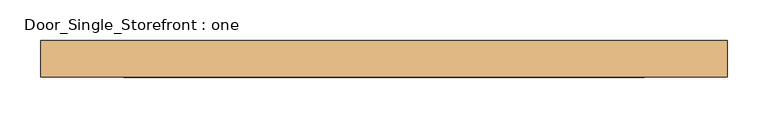
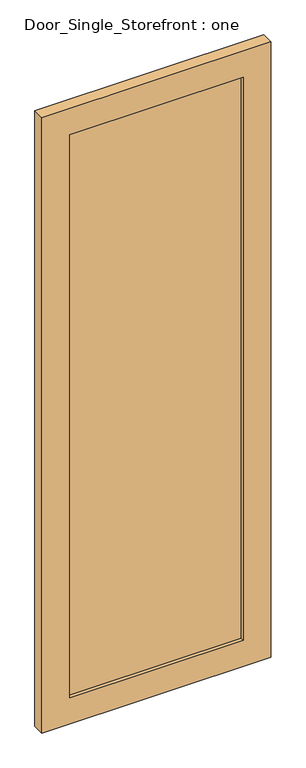
"""IFC4 building model written with IfcOpenShell, lengths in millimetres: door geometry, Door_Single_Storefront : one."""

import ifcopenshell
import ifcopenshell.guid

model = None  # the IFC model being written
_history = None  # IfcOwnerHistory: only IFC2X3 demands one
_inside = {}  # id of a spatial element -> (the spatial element, [elements in it])
_under = {}  # id of a project, library or spatial element -> (it, [spatial elements below it])
_declared = {}  # id of a project -> (the project, [libraries it declares])
_typed = {}  # id of a type object -> (the type object, [elements of that type])
_made_of = {}  # id of a material, layer set ... -> (it, [elements and type objects made of it])


def new_model(schema):
    """Start an empty IFC model of exactly this schema.

    Asked for "IFC4X3", IfcOpenShell would pick the latest addendum, in which some entities
    have other attributes; the version numbers below select the first issue.
    IFC2X3 requires an IfcOwnerHistory on every rooted entity: one is made here for all.
    """
    global model, _history
    if schema == "IFC4X3":
        model = ifcopenshell.file(schema_version=(4, 3, 0, 0))
    else:
        model = ifcopenshell.file(schema=schema)
    _inside.clear()
    _under.clear()
    _declared.clear()
    _typed.clear()
    _made_of.clear()
    _history = None
    if model.schema == "IFC2X3":
        org = make("IfcOrganization", Name="unknown")
        user = make(
            "IfcPersonAndOrganization",
            ThePerson=make("IfcPerson", FamilyName="unknown"),
            TheOrganization=org,
        )
        app = make(
            "IfcApplication",
            ApplicationDeveloper=org,
            Version="unknown",
            ApplicationFullName="unknown",
            ApplicationIdentifier="unknown",
        )
        _history = make(
            "IfcOwnerHistory",
            OwningUser=user,
            OwningApplication=app,
            ChangeAction="ADDED",
            CreationDate=0,
        )
    return model


def make(cls, **values):
    """One entity of the class cls with the attributes given. An attribute that is None is left unset."""
    return model.create_entity(
        cls, **{name: value for name, value in values.items() if value is not None}
    )


def rooted(cls, **values):
    """An entity with a GlobalId (a new one), such as an element, a storey or a relation."""
    return make(cls, GlobalId=ifcopenshell.guid.new(), OwnerHistory=_history, **values)


def si_unit(unit_type, name, prefix=None):
    """IfcSIUnit, for example si_unit("LENGTHUNIT", "METRE", prefix="MILLI")."""
    return make("IfcSIUnit", UnitType=unit_type, Prefix=prefix, Name=name)


def assignment(units):
    """IfcUnitAssignment: the units of a project."""
    return None if units is None else make("IfcUnitAssignment", Units=units)


def point(xyz):
    """IfcCartesianPoint."""
    return None if xyz is None else make("IfcCartesianPoint", Coordinates=xyz)


def direction(xyz):
    """IfcDirection."""
    return None if xyz is None else make("IfcDirection", DirectionRatios=xyz)


def frame(location, z_axis=None, x_axis=None):
    """IfcAxis2Placement3D, a coordinate frame: its origin and axes. An axis left out is left unset."""
    return make(
        "IfcAxis2Placement3D",
        Location=point(location),
        Axis=direction(z_axis),
        RefDirection=direction(x_axis),
    )


def origin():
    """The frame at (0, 0, 0) with its axes left unset."""
    return frame((0.0, 0.0, 0.0))


def place(relative_to, where):
    """IfcLocalPlacement: puts the frame where relative to a parent placement (None: the world)."""
    return make(
        "IfcLocalPlacement", PlacementRelTo=relative_to, RelativePlacement=where
    )


def context(
    kind, dimensions, precision=None, world=None, true_north=None, identifier=None
):
    """IfcGeometricRepresentationContext, for example the 3D "Model" context."""
    return make(
        "IfcGeometricRepresentationContext",
        ContextIdentifier=identifier,
        ContextType=kind,
        CoordinateSpaceDimension=dimensions,
        Precision=precision,
        WorldCoordinateSystem=world,
        TrueNorth=true_north,
    )


def project(units=None, contexts=None):
    """IfcProject with its units and contexts."""
    return rooted(
        "IfcProject",
        Name="project",
        RepresentationContexts=contexts,
        UnitsInContext=assignment(units),
    )


def spatial(cls, under=None, at=None, **own):
    """A site, building, storey or space (cls), placed at a placement, below another one or the project."""
    s = rooted(cls, ObjectPlacement=at, **own)
    if under is not None:
        _under.setdefault(under.id(), (under, []))[1].append(s)
    return s


def polyline(points):
    """IfcPolyline through the points."""
    return make("IfcPolyline", Points=[point(p) for p in points])


def outline(outer, holes=None, kind="AREA"):
    """IfcArbitraryClosedProfileDef: a profile drawn as a closed curve; with holes, ...WithVoids."""
    if holes is None:
        return make("IfcArbitraryClosedProfileDef", ProfileType=kind, OuterCurve=outer)
    return make(
        "IfcArbitraryProfileDefWithVoids",
        ProfileType=kind,
        OuterCurve=outer,
        InnerCurves=holes,
    )


def extrude(swept, where, along, depth):
    """IfcExtrudedAreaSolid: the profile swept, set in the frame where, extruded along a direction by depth."""
    return make(
        "IfcExtrudedAreaSolid",
        SweptArea=swept,
        Position=where,
        ExtrudedDirection=direction(along),
        Depth=depth,
    )


def shape(context_of_items, identifier, shape_type, items):
    """IfcShapeRepresentation: the items that make up one representation, for example the "Body"."""
    return make(
        "IfcShapeRepresentation",
        ContextOfItems=context_of_items,
        RepresentationIdentifier=identifier,
        RepresentationType=shape_type,
        Items=items,
    )


def source(mapping_origin, context_of_items, identifier, shape_type, items):
    """IfcRepresentationMap: a shape defined once, which mapped items show again and again."""
    return make(
        "IfcRepresentationMap",
        MappingOrigin=mapping_origin,
        MappedRepresentation=shape(context_of_items, identifier, shape_type, items),
    )


def transform(
    local_origin,
    x_axis=None,
    y_axis=None,
    z_axis=None,
    scale=None,
    scale2=None,
    scale3=None,
    uniform=True,
):
    """IfcCartesianTransformationOperator3D, or its non-uniform kind. x_axis, y_axis, z_axis: its Axis1, 2, 3."""
    if uniform:
        return make(
            "IfcCartesianTransformationOperator3D",
            Axis1=direction(x_axis),
            Axis2=direction(y_axis),
            LocalOrigin=point(local_origin),
            Scale=scale,
            Axis3=direction(z_axis),
        )
    return make(
        "IfcCartesianTransformationOperator3DnonUniform",
        Axis1=direction(x_axis),
        Axis2=direction(y_axis),
        LocalOrigin=point(local_origin),
        Scale=scale,
        Axis3=direction(z_axis),
        Scale2=scale2,
        Scale3=scale3,
    )


def mapped(mapping_source, mapping_target):
    """IfcMappedItem: shows the shape of a source again, moved by a transform."""
    return make(
        "IfcMappedItem", MappingSource=mapping_source, MappingTarget=mapping_target
    )


def made_of(thing, what):
    """Note that an element or type object is made of a material, layer set ...; save() writes the relation."""
    if what is not None:
        _made_of.setdefault(what.id(), (what, []))[1].append(thing)
    return thing


def element(
    cls,
    number,
    at=None,
    inside=None,
    cuts=None,
    type_object=None,
    material=None,
    context=None,
    identifier="Body",
    shape_type=None,
    held_by="IfcProductDefinitionShape",
    body=None,
    shapes=None,
    **own,
):
    """One element of the class cls, such as IfcWall. Its Tag is "e" and its number.

    at: its placement. inside: the storey or other place that contains it. cuts: it is an
    opening in that element (IfcRelVoidsElement). A single representation is given by context,
    identifier, shape_type and body (its items); several are given by shapes. held_by: the class
    of the entity that holds the representations. save() writes the other relations.
    """
    e = rooted(cls, Tag="e%d" % number, ObjectPlacement=at, **own)
    if body is not None:
        shapes = [shape(context, identifier, shape_type, body)]
    if shapes is not None:
        e.Representation = make(held_by, Representations=shapes)
    if inside is not None:
        _inside.setdefault(inside.id(), (inside, []))[1].append(e)
    if cuts is not None:
        rooted(
            "IfcRelVoidsElement", RelatingBuildingElement=cuts, RelatedOpeningElement=e
        )
    if type_object is not None:
        _typed.setdefault(type_object.id(), (type_object, []))[1].append(e)
    return made_of(e, material)


def aggregate(whole, parts):
    """IfcRelAggregates: a whole, such as a stair, and the parts it consists of."""
    return rooted("IfcRelAggregates", RelatingObject=whole, RelatedObjects=parts)


def save(model, path):
    """Write the relations noted so far, then the file.

    IfcRelAggregates (storeys below a building ...), IfcRelContainedInSpatialStructure (elements
    in a storey), IfcRelDefinesByType, IfcRelAssociatesMaterial and IfcRelDeclares: one each for
    every whole, place, type object, material and project.
    """
    for whole, parts in _under.values():
        aggregate(whole, parts)
    for where, things in _inside.values():
        rooted(
            "IfcRelContainedInSpatialStructure",
            RelatedElements=things,
            RelatingStructure=where,
        )
    for kind, things in _typed.values():
        rooted("IfcRelDefinesByType", RelatedObjects=things, RelatingType=kind)
    for what, things in _made_of.values():
        rooted("IfcRelAssociatesMaterial", RelatedObjects=things, RelatingMaterial=what)
    for by, libraries in _declared.values():
        rooted("IfcRelDeclares", RelatingContext=by, RelatedDefinitions=libraries)
    model.write(path)


def door_single_storefront_one_b47e5b55(model_context):
    return source(origin(), model_context, "Body", "SweptSolid", [
        extrude(outline(polyline([(2387.6, -419.89375), (0.0, -419.89375), (0.0, 419.89375), (2387.6, 419.89375), (2387.6, -419.89375)]), holes=[polyline([(101.6, 318.29375), (101.6, -318.29375), (2286.0, -318.29375), (2286.0, 318.29375), (101.6, 318.29375)])]), frame((0.0, 6.35, 0.0), z_axis=(0.0, 1.0, 0.0), x_axis=(0.0, 0.0, 1.0)), (0.0, 0.0, 1.0), 44.45),
        extrude(outline(polyline([(318.29375, 19.05), (-318.29375, 19.05), (-318.29375, 38.1), (318.29375, 38.1), (318.29375, 19.05)])), frame((0.0, 0.0, 101.6), z_axis=(0.0, 0.0, 1.0), x_axis=(1.0, 0.0, 0.0)), (0.0, 0.0, 1.0), 2184.4),
    ])


if __name__ == "__main__":
    model = new_model("IFC4")
    model_context = context("Model", 3, world=origin())
    ifc_project = project(units=[si_unit("LENGTHUNIT", "METRE", prefix="MILLI")], contexts=[model_context])
    site = spatial("IfcSite", under=ifc_project)
    building = spatial("IfcBuilding", under=site)
    placement = place(None, origin())
    door_single_storefront_one_shape = door_single_storefront_one_b47e5b55(model_context)
    element("IfcDoor", 1, ObjectType="Door_Single_Storefront : one", at=placement, inside=building, context=model_context, shape_type="MappedRepresentation", body=[
        mapped(door_single_storefront_one_shape, transform((0.0, 0.0, 0.0), x_axis=(1.0, 0.0, 0.0), y_axis=(0.0, 1.0, 0.0), z_axis=(0.0, 0.0, 1.0))),
    ])
    save(model, "model.ifc")

# Revit data of these elements
# Type "Door_Single_Storefront : one"
#   Type Mark = "27"
#   Analytic Construction = "<None>"
#   Stile_Width = 0' - 4"
#   Door_Thickness = 0' - 1 3/4"
#   Door_Offset = 0' - 2"
#   Glass_Material = Glass
#   Frame_Material = Aluminum
#   Function = (empty or 0)
# Element 1 (IfcDoor, "Door_Single_Storefront : one")
#   Materials on its faces: "Aluminum", "Glass"
# Materials
#   "Glass": class "Glass", colour RGB 0 128 192, transparency 0.75, Description = "Soda Lime Glass", Cost = 0
#   "Aluminum": class "Metal", colour RGB 247 247 247, transparency 0, Description = "Aluminum 6061", Cost = 0
